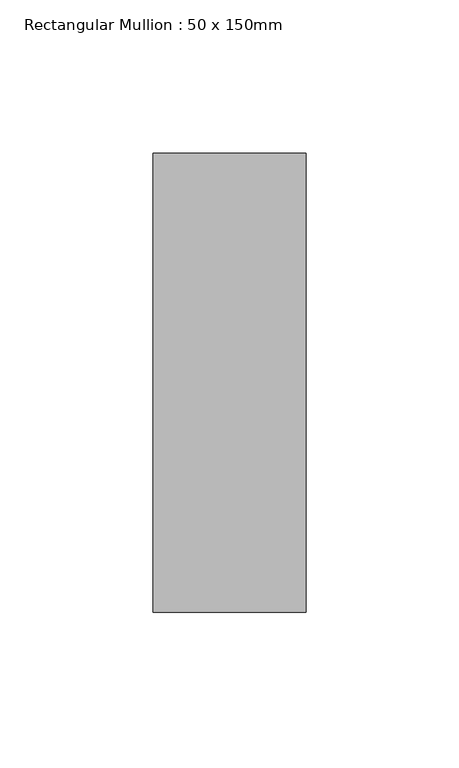
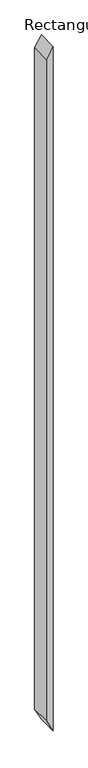
"""IFC4 building model written with IfcOpenShell, lengths in millimetres: member geometry, Rectangular Mullion : 50 x 150mm."""

import ifcopenshell
import ifcopenshell.guid

model = None  # the IFC model being written
_history = None  # IfcOwnerHistory: only IFC2X3 demands one
_inside = {}  # id of a spatial element -> (the spatial element, [elements in it])
_under = {}  # id of a project, library or spatial element -> (it, [spatial elements below it])
_declared = {}  # id of a project -> (the project, [libraries it declares])
_typed = {}  # id of a type object -> (the type object, [elements of that type])
_made_of = {}  # id of a material, layer set ... -> (it, [elements and type objects made of it])


def new_model(schema):
    """Start an empty IFC model of exactly this schema.

    Asked for "IFC4X3", IfcOpenShell would pick the latest addendum, in which some entities
    have other attributes; the version numbers below select the first issue.
    IFC2X3 requires an IfcOwnerHistory on every rooted entity: one is made here for all.
    """
    global model, _history
    if schema == "IFC4X3":
        model = ifcopenshell.file(schema_version=(4, 3, 0, 0))
    else:
        model = ifcopenshell.file(schema=schema)
    _inside.clear()
    _under.clear()
    _declared.clear()
    _typed.clear()
    _made_of.clear()
    _history = None
    if model.schema == "IFC2X3":
        org = make("IfcOrganization", Name="unknown")
        user = make(
            "IfcPersonAndOrganization",
            ThePerson=make("IfcPerson", FamilyName="unknown"),
            TheOrganization=org,
        )
        app = make(
            "IfcApplication",
            ApplicationDeveloper=org,
            Version="unknown",
            ApplicationFullName="unknown",
            ApplicationIdentifier="unknown",
        )
        _history = make(
            "IfcOwnerHistory",
            OwningUser=user,
            OwningApplication=app,
            ChangeAction="ADDED",
            CreationDate=0,
        )
    return model


def make(cls, **values):
    """One entity of the class cls with the attributes given. An attribute that is None is left unset."""
    return model.create_entity(
        cls, **{name: value for name, value in values.items() if value is not None}
    )


def rooted(cls, **values):
    """An entity with a GlobalId (a new one), such as an element, a storey or a relation."""
    return make(cls, GlobalId=ifcopenshell.guid.new(), OwnerHistory=_history, **values)


def si_unit(unit_type, name, prefix=None):
    """IfcSIUnit, for example si_unit("LENGTHUNIT", "METRE", prefix="MILLI")."""
    return make("IfcSIUnit", UnitType=unit_type, Prefix=prefix, Name=name)


def assignment(units):
    """IfcUnitAssignment: the units of a project."""
    return None if units is None else make("IfcUnitAssignment", Units=units)


def point(xyz):
    """IfcCartesianPoint."""
    return None if xyz is None else make("IfcCartesianPoint", Coordinates=xyz)


def direction(xyz):
    """IfcDirection."""
    return None if xyz is None else make("IfcDirection", DirectionRatios=xyz)


def frame(location, z_axis=None, x_axis=None):
    """IfcAxis2Placement3D, a coordinate frame: its origin and axes. An axis left out is left unset."""
    return make(
        "IfcAxis2Placement3D",
        Location=point(location),
        Axis=direction(z_axis),
        RefDirection=direction(x_axis),
    )


def origin():
    """The frame at (0, 0, 0) with its axes left unset."""
    return frame((0.0, 0.0, 0.0))


def place(relative_to, where):
    """IfcLocalPlacement: puts the frame where relative to a parent placement (None: the world)."""
    return make(
        "IfcLocalPlacement", PlacementRelTo=relative_to, RelativePlacement=where
    )


def context(
    kind, dimensions, precision=None, world=None, true_north=None, identifier=None
):
    """IfcGeometricRepresentationContext, for example the 3D "Model" context."""
    return make(
        "IfcGeometricRepresentationContext",
        ContextIdentifier=identifier,
        ContextType=kind,
        CoordinateSpaceDimension=dimensions,
        Precision=precision,
        WorldCoordinateSystem=world,
        TrueNorth=true_north,
    )


def project(units=None, contexts=None):
    """IfcProject with its units and contexts."""
    return rooted(
        "IfcProject",
        Name="project",
        RepresentationContexts=contexts,
        UnitsInContext=assignment(units),
    )


def spatial(cls, under=None, at=None, **own):
    """A site, building, storey or space (cls), placed at a placement, below another one or the project."""
    s = rooted(cls, ObjectPlacement=at, **own)
    if under is not None:
        _under.setdefault(under.id(), (under, []))[1].append(s)
    return s


def polyline(points):
    """IfcPolyline through the points."""
    return make("IfcPolyline", Points=[point(p) for p in points])


def outline(outer, holes=None, kind="AREA"):
    """IfcArbitraryClosedProfileDef: a profile drawn as a closed curve; with holes, ...WithVoids."""
    if holes is None:
        return make("IfcArbitraryClosedProfileDef", ProfileType=kind, OuterCurve=outer)
    return make(
        "IfcArbitraryProfileDefWithVoids",
        ProfileType=kind,
        OuterCurve=outer,
        InnerCurves=holes,
    )


def extrude(swept, where, along, depth):
    """IfcExtrudedAreaSolid: the profile swept, set in the frame where, extruded along a direction by depth."""
    return make(
        "IfcExtrudedAreaSolid",
        SweptArea=swept,
        Position=where,
        ExtrudedDirection=direction(along),
        Depth=depth,
    )


def shape(context_of_items, identifier, shape_type, items):
    """IfcShapeRepresentation: the items that make up one representation, for example the "Body"."""
    return make(
        "IfcShapeRepresentation",
        ContextOfItems=context_of_items,
        RepresentationIdentifier=identifier,
        RepresentationType=shape_type,
        Items=items,
    )


def source(mapping_origin, context_of_items, identifier, shape_type, items):
    """IfcRepresentationMap: a shape defined once, which mapped items show again and again."""
    return make(
        "IfcRepresentationMap",
        MappingOrigin=mapping_origin,
        MappedRepresentation=shape(context_of_items, identifier, shape_type, items),
    )


def transform(
    local_origin,
    x_axis=None,
    y_axis=None,
    z_axis=None,
    scale=None,
    scale2=None,
    scale3=None,
    uniform=True,
):
    """IfcCartesianTransformationOperator3D, or its non-uniform kind. x_axis, y_axis, z_axis: its Axis1, 2, 3."""
    if uniform:
        return make(
            "IfcCartesianTransformationOperator3D",
            Axis1=direction(x_axis),
            Axis2=direction(y_axis),
            LocalOrigin=point(local_origin),
            Scale=scale,
            Axis3=direction(z_axis),
        )
    return make(
        "IfcCartesianTransformationOperator3DnonUniform",
        Axis1=direction(x_axis),
        Axis2=direction(y_axis),
        LocalOrigin=point(local_origin),
        Scale=scale,
        Axis3=direction(z_axis),
        Scale2=scale2,
        Scale3=scale3,
    )


def mapped(mapping_source, mapping_target):
    """IfcMappedItem: shows the shape of a source again, moved by a transform."""
    return make(
        "IfcMappedItem", MappingSource=mapping_source, MappingTarget=mapping_target
    )


def made_of(thing, what):
    """Note that an element or type object is made of a material, layer set ...; save() writes the relation."""
    if what is not None:
        _made_of.setdefault(what.id(), (what, []))[1].append(thing)
    return thing


def element(
    cls,
    number,
    at=None,
    inside=None,
    cuts=None,
    type_object=None,
    material=None,
    context=None,
    identifier="Body",
    shape_type=None,
    held_by="IfcProductDefinitionShape",
    body=None,
    shapes=None,
    **own,
):
    """One element of the class cls, such as IfcWall. Its Tag is "e" and its number.

    at: its placement. inside: the storey or other place that contains it. cuts: it is an
    opening in that element (IfcRelVoidsElement). A single representation is given by context,
    identifier, shape_type and body (its items); several are given by shapes. held_by: the class
    of the entity that holds the representations. save() writes the other relations.
    """
    e = rooted(cls, Tag="e%d" % number, ObjectPlacement=at, **own)
    if body is not None:
        shapes = [shape(context, identifier, shape_type, body)]
    if shapes is not None:
        e.Representation = make(held_by, Representations=shapes)
    if inside is not None:
        _inside.setdefault(inside.id(), (inside, []))[1].append(e)
    if cuts is not None:
        rooted(
            "IfcRelVoidsElement", RelatingBuildingElement=cuts, RelatedOpeningElement=e
        )
    if type_object is not None:
        _typed.setdefault(type_object.id(), (type_object, []))[1].append(e)
    return made_of(e, material)


def aggregate(whole, parts):
    """IfcRelAggregates: a whole, such as a stair, and the parts it consists of."""
    return rooted("IfcRelAggregates", RelatingObject=whole, RelatedObjects=parts)


def save(model, path):
    """Write the relations noted so far, then the file.

    IfcRelAggregates (storeys below a building ...), IfcRelContainedInSpatialStructure (elements
    in a storey), IfcRelDefinesByType, IfcRelAssociatesMaterial and IfcRelDeclares: one each for
    every whole, place, type object, material and project.
    """
    for whole, parts in _under.values():
        aggregate(whole, parts)
    for where, things in _inside.values():
        rooted(
            "IfcRelContainedInSpatialStructure",
            RelatedElements=things,
            RelatingStructure=where,
        )
    for kind, things in _typed.values():
        rooted("IfcRelDefinesByType", RelatedObjects=things, RelatingType=kind)
    for what, things in _made_of.values():
        rooted("IfcRelAssociatesMaterial", RelatedObjects=things, RelatingMaterial=what)
    for by, libraries in _declared.values():
        rooted("IfcRelDeclares", RelatingContext=by, RelatedDefinitions=libraries)
    model.write(path)


def rectangular_mullion_50_x_150mm_72219edf(model_context):
    return source(origin(), model_context, "Body", "SweptSolid", [
        extrude(outline(polyline([(0.0, 0.0), (-83.6497392, -50.0), (-5243.3853965, -50.0), (-5340.1430845, 0.0), (0.0, 0.0)])), frame((0.0, -75.0, 0.0), z_axis=(0.0, 1.0, 0.0), x_axis=(0.0, 0.0, 1.0)), (0.0, 0.0, 1.0), 150.0),
    ])


if __name__ == "__main__":
    model = new_model("IFC4")
    model_context = context("Model", 3, world=origin())
    ifc_project = project(units=[si_unit("LENGTHUNIT", "METRE", prefix="MILLI")], contexts=[model_context])
    site = spatial("IfcSite", under=ifc_project)
    building = spatial("IfcBuilding", under=site)
    placement = place(None, origin())
    rectangular_mullion_50_x_150mm_shape = rectangular_mullion_50_x_150mm_72219edf(model_context)
    element("IfcMember", 1, ObjectType="Rectangular Mullion : 50 x 150mm", at=placement, inside=building, context=model_context, shape_type="MappedRepresentation", body=[
        mapped(rectangular_mullion_50_x_150mm_shape, transform((0.0, 0.0, 0.0), x_axis=(1.0, 0.0, 0.0), y_axis=(0.0, 1.0, 0.0), z_axis=(0.0, 0.0, 1.0))),
    ])
    save(model, "model.ifc")

# Revit data of these elements
# Type "Rectangular Mullion : 50 x 150mm"
#   built-in parameter 1007304 = 0.492126 (stored number, unit not read)
#   built-in parameter 1007301 = 0.082021 (stored number, unit not read)
#   built-in parameter 1007300 = 0.082021 (stored number, unit not read)
# Element 1 (IfcMember, "Rectangular Mullion : 50 x 150mm")
#   Materials on its faces: "Metal - Aluminium"
# Materials
#   "Metal - Aluminium": class "Metal", colour RGB 247 247 247, transparency 0
